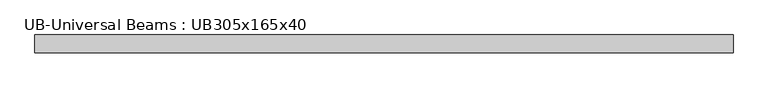
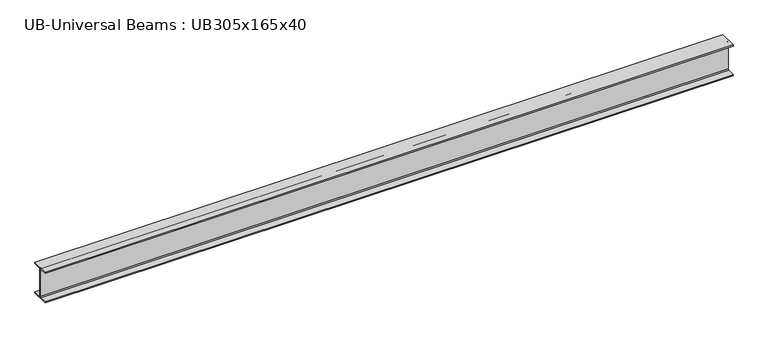
"""IFC4 building model written with IfcOpenShell, lengths in millimetres: beam geometry, UB-Universal Beams : UB305x165x40."""

from ifc_helpers import new_model, si_unit, point, frame, frame_2d, origin, place, context, project, spatial, polyline, circle_curve, trimmed, segment, composite_curve, outline, extrude, source, transform, mapped, element, save


def ub_universal_beams_ub305x165x40_614cc3fe(model_context):
    return source(origin(), model_context, "Body", "SweptSolid", [
        extrude(outline(composite_curve([segment(polyline([(82.5, -141.5), (82.5, -151.7), (-82.5, -151.7), (-82.5, -141.5), (-11.9, -141.5)]), True, "CONTINUOUS"), segment(trimmed(circle_curve(frame_2d((-11.9, -132.6)), 8.9), [point((-11.9, -141.5))], [point((-3.0, -132.6))], True, "CARTESIAN"), True, "CONTINUOUS"), segment(polyline([(-3.0, -132.6), (-3.0, 132.6)]), True, "CONTINUOUS"), segment(trimmed(circle_curve(frame_2d((-11.9, 132.6)), 8.9), [point((-3.0, 132.6))], [point((-11.9, 141.5))], True, "CARTESIAN"), True, "CONTINUOUS"), segment(polyline([(-11.9, 141.5), (-82.5, 141.5), (-82.5, 151.7), (82.5, 151.7), (82.5, 141.5), (11.9, 141.5)]), True, "CONTINUOUS"), segment(trimmed(circle_curve(frame_2d((11.9, 132.6)), 8.9), [point((11.9, 141.5))], [point((3.0, 132.6))], True, "CARTESIAN"), True, "CONTINUOUS"), segment(polyline([(3.0, 132.6), (3.0, -132.6)]), True, "CONTINUOUS"), segment(trimmed(circle_curve(frame_2d((11.9, -132.6)), 8.9), [point((3.0, -132.6))], [point((11.9, -141.5))], True, "CARTESIAN"), True, "CONTINUOUS"), segment(polyline([(11.9, -141.5), (82.5, -141.5)]), True, "CONTINUOUS")], self_intersect=False)), frame((-3226.45, 0.0, 0.0), z_axis=(1.0, 0.0, 0.0), x_axis=(0.0, 1.0, 0.0)), (0.0, 0.0, 1.0), 6452.9),
    ])


if __name__ == "__main__":
    model = new_model("IFC4")
    model_context = context("Model", 3, world=origin())
    ifc_project = project(units=[si_unit("LENGTHUNIT", "METRE", prefix="MILLI")], contexts=[model_context])
    site = spatial("IfcSite", under=ifc_project)
    building = spatial("IfcBuilding", under=site)
    placement = place(None, origin())
    ub_universal_beams_ub305x165x40_shape = ub_universal_beams_ub305x165x40_614cc3fe(model_context)
    element("IfcBeam", 1, ObjectType="UB-Universal Beams : UB305x165x40", at=placement, inside=building, context=model_context, shape_type="MappedRepresentation", body=[
        mapped(ub_universal_beams_ub305x165x40_shape, transform((0.0, 0.0, 0.0), x_axis=(1.0, 0.0, 0.0), y_axis=(0.0, 1.0, 0.0), z_axis=(0.0, 0.0, 1.0))),
    ])
    save(model, "model.ifc")

# Revit data of these elements
# Type "UB-Universal Beams : UB305x165x40"
#   Section Name Key = "UB305X165X40"
#   Width = 16.5 cm
#   Web Thickness = 0.6 cm
#   Web Fillet = 0.89 cm
#   Warping Constant = 164000.0 cm⁶
#   Torsional Moment of Inertia = 14.70 cm⁴
#   Section Area = 51.3 cm²
#   Plastic Modulus weak axis = 142.0 cm³
#   Plastic Modulus strong axis = 623.0 cm³
#   Nominal Weight = 40.2999 kgf/m
#   Moment of Inertia weak axis = 764.00 cm⁴
#   Moment of Inertia strong axis = 8503.00 cm⁴
#   Height = 30.34 cm
#   Flange Thickness = 1.02 cm
#   Elastic Modulus weak axis = 92.6 cm³
#   Elastic Modulus strong axis = 560.0 cm³
#   Centroid Vertical = 15.17 cm
#   Centroid Horizontal = 8.25 cm
#   Bolt Spacing = 9.0 cm
#   Length [instance default] = 1500 mm
#   Structural Material [instance default] = Metal - Steel 43-275
#   Type Comments = ""
#   Assembly Code = ""
# Element 1 (IfcBeam, "UB-Universal Beams : UB305x165x40")
#   Materials on its faces: "Metal - Steel 43-275"
# Materials
#   "Metal - Steel 43-275": class "Metal", colour RGB 247 247 247, transparency 0, Cost = 0
